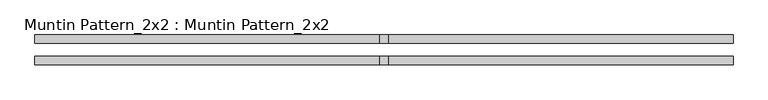
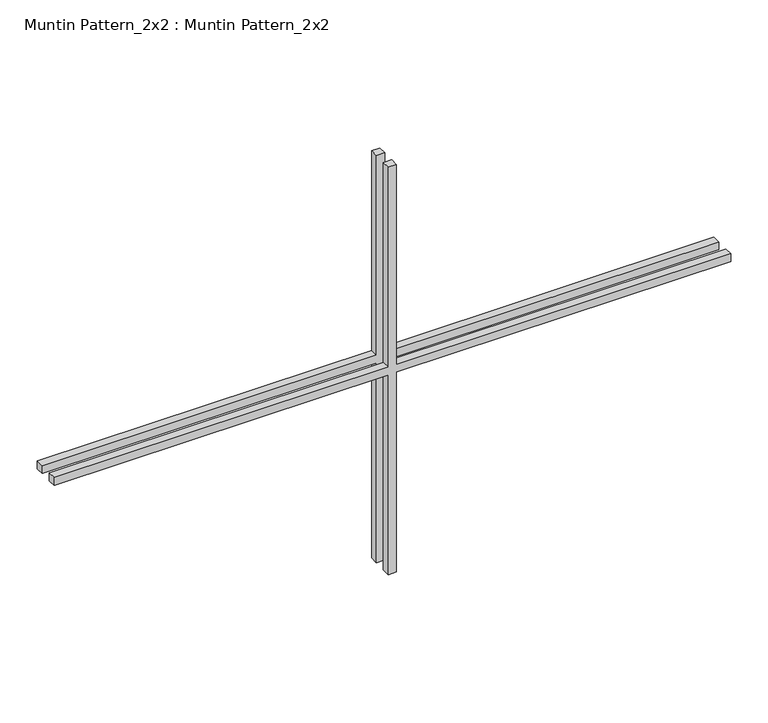
"""IFC4 building model written with IfcOpenShell, lengths in millimetres: proxy geometry, Muntin Pattern_2x2 : Muntin Pattern_2x2."""

import ifcopenshell
import ifcopenshell.guid

model = None  # the IFC model being written
_history = None  # IfcOwnerHistory: only IFC2X3 demands one
_inside = {}  # id of a spatial element -> (the spatial element, [elements in it])
_under = {}  # id of a project, library or spatial element -> (it, [spatial elements below it])
_declared = {}  # id of a project -> (the project, [libraries it declares])
_typed = {}  # id of a type object -> (the type object, [elements of that type])
_made_of = {}  # id of a material, layer set ... -> (it, [elements and type objects made of it])


def new_model(schema):
    """Start an empty IFC model of exactly this schema.

    Asked for "IFC4X3", IfcOpenShell would pick the latest addendum, in which some entities
    have other attributes; the version numbers below select the first issue.
    IFC2X3 requires an IfcOwnerHistory on every rooted entity: one is made here for all.
    """
    global model, _history
    if schema == "IFC4X3":
        model = ifcopenshell.file(schema_version=(4, 3, 0, 0))
    else:
        model = ifcopenshell.file(schema=schema)
    _inside.clear()
    _under.clear()
    _declared.clear()
    _typed.clear()
    _made_of.clear()
    _history = None
    if model.schema == "IFC2X3":
        org = make("IfcOrganization", Name="unknown")
        user = make(
            "IfcPersonAndOrganization",
            ThePerson=make("IfcPerson", FamilyName="unknown"),
            TheOrganization=org,
        )
        app = make(
            "IfcApplication",
            ApplicationDeveloper=org,
            Version="unknown",
            ApplicationFullName="unknown",
            ApplicationIdentifier="unknown",
        )
        _history = make(
            "IfcOwnerHistory",
            OwningUser=user,
            OwningApplication=app,
            ChangeAction="ADDED",
            CreationDate=0,
        )
    return model


def make(cls, **values):
    """One entity of the class cls with the attributes given. An attribute that is None is left unset."""
    return model.create_entity(
        cls, **{name: value for name, value in values.items() if value is not None}
    )


def rooted(cls, **values):
    """An entity with a GlobalId (a new one), such as an element, a storey or a relation."""
    return make(cls, GlobalId=ifcopenshell.guid.new(), OwnerHistory=_history, **values)


def si_unit(unit_type, name, prefix=None):
    """IfcSIUnit, for example si_unit("LENGTHUNIT", "METRE", prefix="MILLI")."""
    return make("IfcSIUnit", UnitType=unit_type, Prefix=prefix, Name=name)


def assignment(units):
    """IfcUnitAssignment: the units of a project."""
    return None if units is None else make("IfcUnitAssignment", Units=units)


def point(xyz):
    """IfcCartesianPoint."""
    return None if xyz is None else make("IfcCartesianPoint", Coordinates=xyz)


def direction(xyz):
    """IfcDirection."""
    return None if xyz is None else make("IfcDirection", DirectionRatios=xyz)


def frame(location, z_axis=None, x_axis=None):
    """IfcAxis2Placement3D, a coordinate frame: its origin and axes. An axis left out is left unset."""
    return make(
        "IfcAxis2Placement3D",
        Location=point(location),
        Axis=direction(z_axis),
        RefDirection=direction(x_axis),
    )


def origin():
    """The frame at (0, 0, 0) with its axes left unset."""
    return frame((0.0, 0.0, 0.0))


def place(relative_to, where):
    """IfcLocalPlacement: puts the frame where relative to a parent placement (None: the world)."""
    return make(
        "IfcLocalPlacement", PlacementRelTo=relative_to, RelativePlacement=where
    )


def context(
    kind, dimensions, precision=None, world=None, true_north=None, identifier=None
):
    """IfcGeometricRepresentationContext, for example the 3D "Model" context."""
    return make(
        "IfcGeometricRepresentationContext",
        ContextIdentifier=identifier,
        ContextType=kind,
        CoordinateSpaceDimension=dimensions,
        Precision=precision,
        WorldCoordinateSystem=world,
        TrueNorth=true_north,
    )


def project(units=None, contexts=None):
    """IfcProject with its units and contexts."""
    return rooted(
        "IfcProject",
        Name="project",
        RepresentationContexts=contexts,
        UnitsInContext=assignment(units),
    )


def spatial(cls, under=None, at=None, **own):
    """A site, building, storey or space (cls), placed at a placement, below another one or the project."""
    s = rooted(cls, ObjectPlacement=at, **own)
    if under is not None:
        _under.setdefault(under.id(), (under, []))[1].append(s)
    return s


def polyline(points):
    """IfcPolyline through the points."""
    return make("IfcPolyline", Points=[point(p) for p in points])


def outline(outer, holes=None, kind="AREA"):
    """IfcArbitraryClosedProfileDef: a profile drawn as a closed curve; with holes, ...WithVoids."""
    if holes is None:
        return make("IfcArbitraryClosedProfileDef", ProfileType=kind, OuterCurve=outer)
    return make(
        "IfcArbitraryProfileDefWithVoids",
        ProfileType=kind,
        OuterCurve=outer,
        InnerCurves=holes,
    )


def extrude(swept, where, along, depth):
    """IfcExtrudedAreaSolid: the profile swept, set in the frame where, extruded along a direction by depth."""
    return make(
        "IfcExtrudedAreaSolid",
        SweptArea=swept,
        Position=where,
        ExtrudedDirection=direction(along),
        Depth=depth,
    )


def shape(context_of_items, identifier, shape_type, items):
    """IfcShapeRepresentation: the items that make up one representation, for example the "Body"."""
    return make(
        "IfcShapeRepresentation",
        ContextOfItems=context_of_items,
        RepresentationIdentifier=identifier,
        RepresentationType=shape_type,
        Items=items,
    )


def source(mapping_origin, context_of_items, identifier, shape_type, items):
    """IfcRepresentationMap: a shape defined once, which mapped items show again and again."""
    return make(
        "IfcRepresentationMap",
        MappingOrigin=mapping_origin,
        MappedRepresentation=shape(context_of_items, identifier, shape_type, items),
    )


def transform(
    local_origin,
    x_axis=None,
    y_axis=None,
    z_axis=None,
    scale=None,
    scale2=None,
    scale3=None,
    uniform=True,
):
    """IfcCartesianTransformationOperator3D, or its non-uniform kind. x_axis, y_axis, z_axis: its Axis1, 2, 3."""
    if uniform:
        return make(
            "IfcCartesianTransformationOperator3D",
            Axis1=direction(x_axis),
            Axis2=direction(y_axis),
            LocalOrigin=point(local_origin),
            Scale=scale,
            Axis3=direction(z_axis),
        )
    return make(
        "IfcCartesianTransformationOperator3DnonUniform",
        Axis1=direction(x_axis),
        Axis2=direction(y_axis),
        LocalOrigin=point(local_origin),
        Scale=scale,
        Axis3=direction(z_axis),
        Scale2=scale2,
        Scale3=scale3,
    )


def mapped(mapping_source, mapping_target):
    """IfcMappedItem: shows the shape of a source again, moved by a transform."""
    return make(
        "IfcMappedItem", MappingSource=mapping_source, MappingTarget=mapping_target
    )


def made_of(thing, what):
    """Note that an element or type object is made of a material, layer set ...; save() writes the relation."""
    if what is not None:
        _made_of.setdefault(what.id(), (what, []))[1].append(thing)
    return thing


def element(
    cls,
    number,
    at=None,
    inside=None,
    cuts=None,
    type_object=None,
    material=None,
    context=None,
    identifier="Body",
    shape_type=None,
    held_by="IfcProductDefinitionShape",
    body=None,
    shapes=None,
    **own,
):
    """One element of the class cls, such as IfcWall. Its Tag is "e" and its number.

    at: its placement. inside: the storey or other place that contains it. cuts: it is an
    opening in that element (IfcRelVoidsElement). A single representation is given by context,
    identifier, shape_type and body (its items); several are given by shapes. held_by: the class
    of the entity that holds the representations. save() writes the other relations.
    """
    e = rooted(cls, Tag="e%d" % number, ObjectPlacement=at, **own)
    if body is not None:
        shapes = [shape(context, identifier, shape_type, body)]
    if shapes is not None:
        e.Representation = make(held_by, Representations=shapes)
    if inside is not None:
        _inside.setdefault(inside.id(), (inside, []))[1].append(e)
    if cuts is not None:
        rooted(
            "IfcRelVoidsElement", RelatingBuildingElement=cuts, RelatedOpeningElement=e
        )
    if type_object is not None:
        _typed.setdefault(type_object.id(), (type_object, []))[1].append(e)
    return made_of(e, material)


def aggregate(whole, parts):
    """IfcRelAggregates: a whole, such as a stair, and the parts it consists of."""
    return rooted("IfcRelAggregates", RelatingObject=whole, RelatedObjects=parts)


def save(model, path):
    """Write the relations noted so far, then the file.

    IfcRelAggregates (storeys below a building ...), IfcRelContainedInSpatialStructure (elements
    in a storey), IfcRelDefinesByType, IfcRelAssociatesMaterial and IfcRelDeclares: one each for
    every whole, place, type object, material and project.
    """
    for whole, parts in _under.values():
        aggregate(whole, parts)
    for where, things in _inside.values():
        rooted(
            "IfcRelContainedInSpatialStructure",
            RelatedElements=things,
            RelatingStructure=where,
        )
    for kind, things in _typed.values():
        rooted("IfcRelDefinesByType", RelatedObjects=things, RelatingType=kind)
    for what, things in _made_of.values():
        rooted("IfcRelAssociatesMaterial", RelatedObjects=things, RelatingMaterial=what)
    for by, libraries in _declared.values():
        rooted("IfcRelDeclares", RelatingContext=by, RelatedDefinitions=libraries)
    model.write(path)


def muntin_pattern_2x2_muntin_pattern_2x2_872d1288(model_context):
    return source(origin(), model_context, "Body", "SweptSolid", [
        extrude(outline(polyline([(338.1375, -6.35), (338.1375, -520.7), (325.4375, -520.7), (325.4375, -6.35), (0.0, -6.35), (0.0, 6.35), (325.4375, 6.35), (325.4375, 520.7), (338.1375, 520.7), (338.1375, 6.35), (663.575, 6.35), (663.575, -6.35), (338.1375, -6.35)])), frame((0.0, 9.525, 0.0), z_axis=(0.0, 1.0, 0.0), x_axis=(0.0, 0.0, 1.0)), (0.0, 0.0, 1.0), 12.7),
        extrude(outline(polyline([(338.1375, -6.35), (338.1375, -520.7), (325.4375, -520.7), (325.4375, -6.35), (0.0, -6.35), (0.0, 6.35), (325.4375, 6.35), (325.4375, 520.7), (338.1375, 520.7), (338.1375, 6.35), (663.575, 6.35), (663.575, -6.35), (338.1375, -6.35)])), frame((0.0, -22.225, 0.0), z_axis=(0.0, 1.0, 0.0), x_axis=(0.0, 0.0, 1.0)), (0.0, 0.0, 1.0), 12.7),
    ])


if __name__ == "__main__":
    model = new_model("IFC4")
    model_context = context("Model", 3, world=origin())
    ifc_project = project(units=[si_unit("LENGTHUNIT", "METRE", prefix="MILLI")], contexts=[model_context])
    site = spatial("IfcSite", under=ifc_project)
    building = spatial("IfcBuilding", under=site)
    placement = place(None, origin())
    muntin_pattern_2x2_muntin_pattern_2x2_shape = muntin_pattern_2x2_muntin_pattern_2x2_872d1288(model_context)
    element("IfcBuildingElementProxy", 1, Name="Muntin Pattern_2x2 : Muntin Pattern_2x2", ObjectType="Muntin Pattern_2x2 : Muntin Pattern_2x2", at=placement, inside=building, context=model_context, shape_type="MappedRepresentation", body=[
        mapped(muntin_pattern_2x2_muntin_pattern_2x2_shape, transform((0.0, 0.0, 0.0), x_axis=(1.0, 0.0, 0.0), y_axis=(0.0, 1.0, 0.0), z_axis=(0.0, 0.0, 1.0))),
    ])
    save(model, "model.ifc")

# Revit data of these elements
# Type "Muntin Pattern_2x2 : Muntin Pattern_2x2"
#   Width [instance default] = 4' - 0"
#   Thickness = 0' - 0 1/2"
#   Height [instance default] = 4' - 0"
#   Distance = 0' - 0 3/4"
#   Interior Material [instance default] = none
#   Exterior Material [instance default] = none
#   Default Elevation = 0
# Element 1 (IfcBuildingElementProxy, "Muntin Pattern_2x2 : Muntin Pattern_2x2")
#   Width = 3' - 5"
#   Height = 2' - 2 1/8"
#   Interior Material = Wood - Stained
#   Exterior Material = Clad - White
#   Materials on its faces: "Clad - White", "Wood - Stained"
# Materials
#   "Clad - White": class "Wood", colour RGB 242 242 238, transparency 0, Cost = 0
#   "Wood - Stained": class "Wood", colour RGB 224 178 126, transparency 0, Cost = 0
